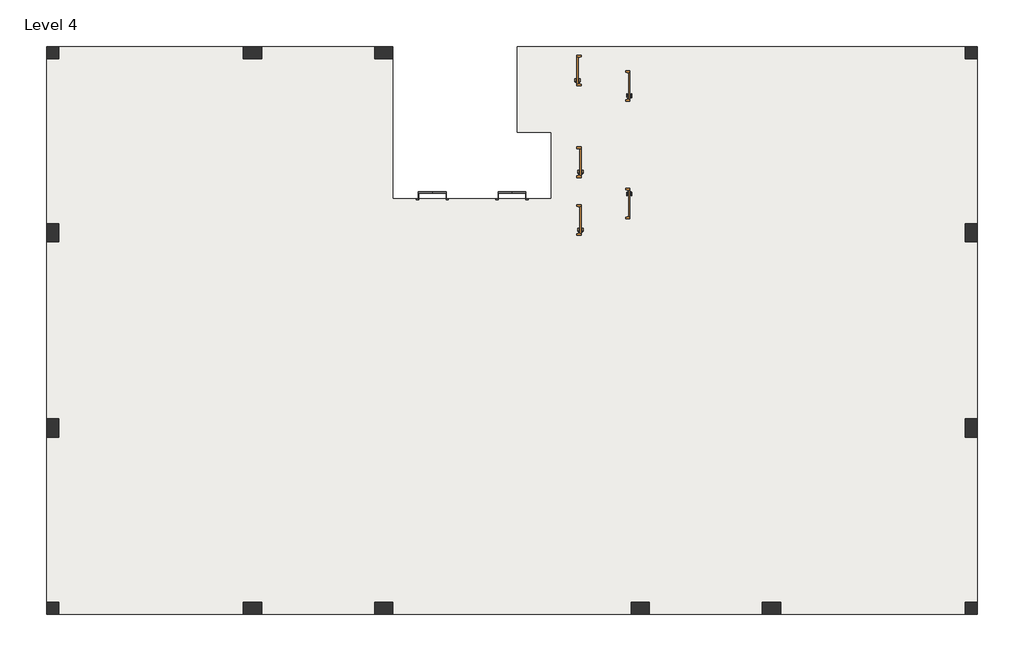
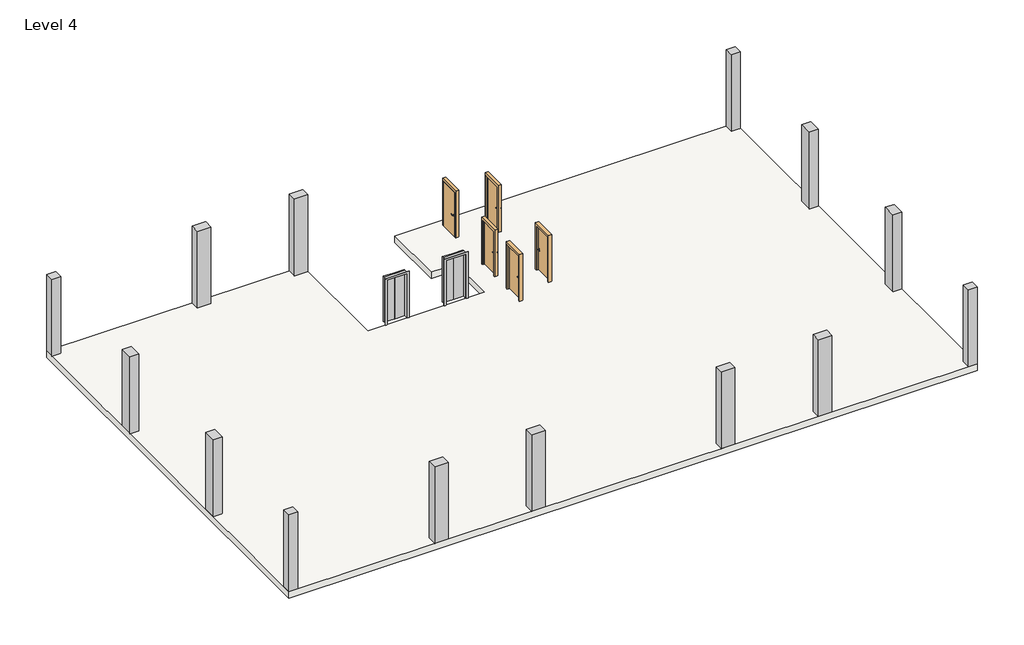
# One storey: 14 columns, 5 doors, 2 proxies, 1 slab.
"""IFC4 building model written with IfcOpenShell, lengths in millimetres."""

import ifcopenshell
import ifcopenshell.guid

model = None  # the IFC model being written
_history = None  # IfcOwnerHistory: only IFC2X3 demands one
_inside = {}  # id of a spatial element -> (the spatial element, [elements in it])
_under = {}  # id of a project, library or spatial element -> (it, [spatial elements below it])
_declared = {}  # id of a project -> (the project, [libraries it declares])
_typed = {}  # id of a type object -> (the type object, [elements of that type])
_made_of = {}  # id of a material, layer set ... -> (it, [elements and type objects made of it])


def new_model(schema):
    """Start an empty IFC model of exactly this schema.

    Asked for "IFC4X3", IfcOpenShell would pick the latest addendum, in which some entities
    have other attributes; the version numbers below select the first issue.
    IFC2X3 requires an IfcOwnerHistory on every rooted entity: one is made here for all.
    """
    global model, _history
    if schema == "IFC4X3":
        model = ifcopenshell.file(schema_version=(4, 3, 0, 0))
    else:
        model = ifcopenshell.file(schema=schema)
    _inside.clear()
    _under.clear()
    _declared.clear()
    _typed.clear()
    _made_of.clear()
    _history = None
    if model.schema == "IFC2X3":
        org = make("IfcOrganization", Name="unknown")
        user = make(
            "IfcPersonAndOrganization",
            ThePerson=make("IfcPerson", FamilyName="unknown"),
            TheOrganization=org,
        )
        app = make(
            "IfcApplication",
            ApplicationDeveloper=org,
            Version="unknown",
            ApplicationFullName="unknown",
            ApplicationIdentifier="unknown",
        )
        _history = make(
            "IfcOwnerHistory",
            OwningUser=user,
            OwningApplication=app,
            ChangeAction="ADDED",
            CreationDate=0,
        )
    return model


def make(cls, **values):
    """One entity of the class cls with the attributes given. An attribute that is None is left unset."""
    return model.create_entity(
        cls, **{name: value for name, value in values.items() if value is not None}
    )


def rooted(cls, **values):
    """An entity with a GlobalId (a new one), such as an element, a storey or a relation."""
    return make(cls, GlobalId=ifcopenshell.guid.new(), OwnerHistory=_history, **values)


def si_unit(unit_type, name, prefix=None):
    """IfcSIUnit, for example si_unit("LENGTHUNIT", "METRE", prefix="MILLI")."""
    return make("IfcSIUnit", UnitType=unit_type, Prefix=prefix, Name=name)


def assignment(units):
    """IfcUnitAssignment: the units of a project."""
    return None if units is None else make("IfcUnitAssignment", Units=units)


def point(xyz):
    """IfcCartesianPoint."""
    return None if xyz is None else make("IfcCartesianPoint", Coordinates=xyz)


def direction(xyz):
    """IfcDirection."""
    return None if xyz is None else make("IfcDirection", DirectionRatios=xyz)


def frame(location, z_axis=None, x_axis=None):
    """IfcAxis2Placement3D, a coordinate frame: its origin and axes. An axis left out is left unset."""
    return make(
        "IfcAxis2Placement3D",
        Location=point(location),
        Axis=direction(z_axis),
        RefDirection=direction(x_axis),
    )


def frame_2d(location, x_axis=None):
    """IfcAxis2Placement2D, a coordinate frame in the plane: its origin and x axis."""
    return make(
        "IfcAxis2Placement2D", Location=point(location), RefDirection=direction(x_axis)
    )


def origin():
    """The frame at (0, 0, 0) with its axes left unset."""
    return frame((0.0, 0.0, 0.0))


def origin_with_axes():
    """The frame at (0, 0, 0) with the z axis (0, 0, 1) and the x axis (1, 0, 0) written out."""
    return frame((0.0, 0.0, 0.0), z_axis=(0.0, 0.0, 1.0), x_axis=(1.0, 0.0, 0.0))


def place(relative_to, where):
    """IfcLocalPlacement: puts the frame where relative to a parent placement (None: the world)."""
    return make(
        "IfcLocalPlacement", PlacementRelTo=relative_to, RelativePlacement=where
    )


def context(
    kind, dimensions, precision=None, world=None, true_north=None, identifier=None
):
    """IfcGeometricRepresentationContext, for example the 3D "Model" context."""
    return make(
        "IfcGeometricRepresentationContext",
        ContextIdentifier=identifier,
        ContextType=kind,
        CoordinateSpaceDimension=dimensions,
        Precision=precision,
        WorldCoordinateSystem=world,
        TrueNorth=true_north,
    )


def project(units=None, contexts=None):
    """IfcProject with its units and contexts."""
    return rooted(
        "IfcProject",
        Name="project",
        RepresentationContexts=contexts,
        UnitsInContext=assignment(units),
    )


def spatial(cls, under=None, at=None, **own):
    """A site, building, storey or space (cls), placed at a placement, below another one or the project."""
    s = rooted(cls, ObjectPlacement=at, **own)
    if under is not None:
        _under.setdefault(under.id(), (under, []))[1].append(s)
    return s


def polyline(points):
    """IfcPolyline through the points."""
    return make("IfcPolyline", Points=[point(p) for p in points])


def circle_curve(where, radius):
    """IfcCircle in the frame where."""
    return make("IfcCircle", Position=where, Radius=radius)


def ellipse_curve(where, semi_axis1, semi_axis2):
    """IfcEllipse in the frame where."""
    return make(
        "IfcEllipse", Position=where, SemiAxis1=semi_axis1, SemiAxis2=semi_axis2
    )


def trimmed(basis, trim1, trim2, sense, master):
    """IfcTrimmedCurve: the piece of a basis curve between two trims."""
    return make(
        "IfcTrimmedCurve",
        BasisCurve=basis,
        Trim1=trim1,
        Trim2=trim2,
        SenseAgreement=sense,
        MasterRepresentation=master,
    )


def segment(curve, same_sense, transition):
    """IfcCompositeCurveSegment."""
    return make(
        "IfcCompositeCurveSegment",
        Transition=transition,
        SameSense=same_sense,
        ParentCurve=curve,
    )


def composite_curve(segments, self_intersect=None):
    """IfcCompositeCurve: segments joined end to end."""
    return make("IfcCompositeCurve", Segments=segments, SelfIntersect=self_intersect)


def outline(outer, holes=None, kind="AREA"):
    """IfcArbitraryClosedProfileDef: a profile drawn as a closed curve; with holes, ...WithVoids."""
    if holes is None:
        return make("IfcArbitraryClosedProfileDef", ProfileType=kind, OuterCurve=outer)
    return make(
        "IfcArbitraryProfileDefWithVoids",
        ProfileType=kind,
        OuterCurve=outer,
        InnerCurves=holes,
    )


def extrude(swept, where, along, depth):
    """IfcExtrudedAreaSolid: the profile swept, set in the frame where, extruded along a direction by depth."""
    return make(
        "IfcExtrudedAreaSolid",
        SweptArea=swept,
        Position=where,
        ExtrudedDirection=direction(along),
        Depth=depth,
    )


def faces_of(points, faces, orient=None, outer=None):
    """IfcFace entities. A face is a list of loops; a loop is a list of indices into points, from 0.

    orient and outer hold one flag for each loop. By default every Orientation is true, the
    first loop of a face is its IfcFaceOuterBound and the others are IfcFaceBound.
    """
    made = []
    for i, loops in enumerate(faces):
        bounds = []
        for j, loop in enumerate(loops):
            is_outer = j == 0 if outer is None else outer[i][j]
            bounds.append(
                make(
                    "IfcFaceOuterBound" if is_outer else "IfcFaceBound",
                    Bound=make("IfcPolyLoop", Polygon=[points[k] for k in loop]),
                    Orientation=True if orient is None else orient[i][j],
                )
            )
        made.append(make("IfcFace", Bounds=bounds))
    return made


def faceted_brep(points, faces, orient=None, outer=None, voids=None):
    """IfcFacetedBrep: a solid bounded by flat faces; with voids (closed shells), ...WithVoids."""
    shared = [point(p) for p in points]
    hull = make("IfcClosedShell", CfsFaces=faces_of(shared, faces, orient, outer))
    if voids is None:
        return make("IfcFacetedBrep", Outer=hull)
    return make(
        "IfcFacetedBrepWithVoids",
        Outer=hull,
        Voids=[
            make(cls, CfsFaces=faces_of(shared, fs, o, b)) for cls, fs, o, b in voids
        ],
    )


def shape(context_of_items, identifier, shape_type, items):
    """IfcShapeRepresentation: the items that make up one representation, for example the "Body"."""
    return make(
        "IfcShapeRepresentation",
        ContextOfItems=context_of_items,
        RepresentationIdentifier=identifier,
        RepresentationType=shape_type,
        Items=items,
    )


def source(mapping_origin, context_of_items, identifier, shape_type, items):
    """IfcRepresentationMap: a shape defined once, which mapped items show again and again."""
    return make(
        "IfcRepresentationMap",
        MappingOrigin=mapping_origin,
        MappedRepresentation=shape(context_of_items, identifier, shape_type, items),
    )


def transform(
    local_origin,
    x_axis=None,
    y_axis=None,
    z_axis=None,
    scale=None,
    scale2=None,
    scale3=None,
    uniform=True,
):
    """IfcCartesianTransformationOperator3D, or its non-uniform kind. x_axis, y_axis, z_axis: its Axis1, 2, 3."""
    if uniform:
        return make(
            "IfcCartesianTransformationOperator3D",
            Axis1=direction(x_axis),
            Axis2=direction(y_axis),
            LocalOrigin=point(local_origin),
            Scale=scale,
            Axis3=direction(z_axis),
        )
    return make(
        "IfcCartesianTransformationOperator3DnonUniform",
        Axis1=direction(x_axis),
        Axis2=direction(y_axis),
        LocalOrigin=point(local_origin),
        Scale=scale,
        Axis3=direction(z_axis),
        Scale2=scale2,
        Scale3=scale3,
    )


def mapped(mapping_source, mapping_target):
    """IfcMappedItem: shows the shape of a source again, moved by a transform."""
    return make(
        "IfcMappedItem", MappingSource=mapping_source, MappingTarget=mapping_target
    )


def made_of(thing, what):
    """Note that an element or type object is made of a material, layer set ...; save() writes the relation."""
    if what is not None:
        _made_of.setdefault(what.id(), (what, []))[1].append(thing)
    return thing


def element(
    cls,
    number,
    at=None,
    inside=None,
    cuts=None,
    type_object=None,
    material=None,
    context=None,
    identifier="Body",
    shape_type=None,
    held_by="IfcProductDefinitionShape",
    body=None,
    shapes=None,
    **own,
):
    """One element of the class cls, such as IfcWall. Its Tag is "e" and its number.

    at: its placement. inside: the storey or other place that contains it. cuts: it is an
    opening in that element (IfcRelVoidsElement). A single representation is given by context,
    identifier, shape_type and body (its items); several are given by shapes. held_by: the class
    of the entity that holds the representations. save() writes the other relations.
    """
    e = rooted(cls, Tag="e%d" % number, ObjectPlacement=at, **own)
    if body is not None:
        shapes = [shape(context, identifier, shape_type, body)]
    if shapes is not None:
        e.Representation = make(held_by, Representations=shapes)
    if inside is not None:
        _inside.setdefault(inside.id(), (inside, []))[1].append(e)
    if cuts is not None:
        rooted(
            "IfcRelVoidsElement", RelatingBuildingElement=cuts, RelatedOpeningElement=e
        )
    if type_object is not None:
        _typed.setdefault(type_object.id(), (type_object, []))[1].append(e)
    return made_of(e, material)


def aggregate(whole, parts):
    """IfcRelAggregates: a whole, such as a stair, and the parts it consists of."""
    return rooted("IfcRelAggregates", RelatingObject=whole, RelatedObjects=parts)


def save(model, path):
    """Write the relations noted so far, then the file.

    IfcRelAggregates (storeys below a building ...), IfcRelContainedInSpatialStructure (elements
    in a storey), IfcRelDefinesByType, IfcRelAssociatesMaterial and IfcRelDeclares: one each for
    every whole, place, type object, material and project.
    """
    for whole, parts in _under.values():
        aggregate(whole, parts)
    for where, things in _inside.values():
        rooted(
            "IfcRelContainedInSpatialStructure",
            RelatedElements=things,
            RelatingStructure=where,
        )
    for kind, things in _typed.values():
        rooted("IfcRelDefinesByType", RelatedObjects=things, RelatingType=kind)
    for what, things in _made_of.values():
        rooted("IfcRelAssociatesMaterial", RelatedObjects=things, RelatingMaterial=what)
    for by, libraries in _declared.values():
        rooted("IfcRelDeclares", RelatingContext=by, RelatedDefinitions=libraries)
    model.write(path)


def plane_surface(at):
    """IfcPlane: the flat surface through the origin of the frame at, square to its z axis."""
    return make("IfcPlane", Position=at)


def cylinder_surface(at, radius):
    """IfcCylindricalSurface: all points at the distance radius from the z axis of the frame at."""
    return make("IfcCylindricalSurface", Position=at, Radius=radius)


def revolved_surface(curve, axis_point, axis_direction):
    """IfcSurfaceOfRevolution: the curve turned about the line through axis_point along axis_direction."""
    return make(
        "IfcSurfaceOfRevolution",
        SweptCurve=make("IfcArbitraryOpenProfileDef", ProfileType="CURVE", Curve=curve),
        AxisPosition=make("IfcAxis1Placement", Location=point(axis_point), Axis=direction(axis_direction)),
    )


def advanced_brep(points, edges, surfaces, faces):
    """IfcAdvancedBrep: a solid bounded by faces that lie on surfaces and meet in shared edges.

    An edge is (start, end): straight between two places in points (the first is 0);
    or (start, end, curve); or (start, end, curve, False) where it runs against its curve.
    A face is (place in surfaces, loops), or (place, loops, False) where it looks against
    its surface's normal. A loop lists edges by number (the first is 1), with a minus sign
    where the edge is run from its end to its start. The first loop is the outer one.
    """
    corners = [point(p) for p in points]
    vertices = [make("IfcVertexPoint", VertexGeometry=c) for c in corners]
    made = []
    for start, end, *more in edges:
        made.append(
            make(
                "IfcEdgeCurve",
                EdgeStart=vertices[start],
                EdgeEnd=vertices[end],
                EdgeGeometry=more[0] if more else make("IfcPolyline", Points=[corners[start], corners[end]]),
                SameSense=more[1] if len(more) > 1 else True,
            )
        )
    hull = []
    for where, loops, *sense in faces:
        bounds = []
        for j, loop in enumerate(loops):
            ring = [make("IfcOrientedEdge", EdgeElement=made[abs(k) - 1], Orientation=k > 0) for k in loop]
            bounds.append(
                make(
                    "IfcFaceOuterBound" if j == 0 else "IfcFaceBound",
                    Bound=make("IfcEdgeLoop", EdgeList=ring),
                    Orientation=True,
                )
            )
        hull.append(make("IfcAdvancedFace", Bounds=bounds, FaceSurface=surfaces[where], SameSense=sense[0] if sense else True))
    return make("IfcAdvancedBrep", Outer=make("IfcClosedShell", CfsFaces=hull))


def proxy_71d7088b(model_context):
    return source(origin(), model_context, "Body", "SweptSolid", [
        extrude(outline(polyline([(-102.3106443, 96.8375), (-562.6856443, 96.8375), (-562.6856443, 147.6375), (-102.3106443, 147.6375), (-102.3106443, 96.8375)])), origin_with_axes(), (0.0, 0.0, 1.0), 2159.0),
        extrude(outline(polyline([(364.4143557, 96.8375), (-95.9606443, 96.8375), (-95.9606443, 147.6375), (364.4143557, 147.6375), (364.4143557, 96.8375)])), origin_with_axes(), (0.0, 0.0, 1.0), 2159.0),
        extrude(outline(polyline([(0.0, -562.6856443), (0.0, -556.3356443), (2133.6, -556.3356443), (2133.6, 358.0643557), (0.0, 358.0643557), (0.0, 364.4143557), (2159.0, 364.4143557), (2159.0, -562.6856443), (0.0, -562.6856443)])), frame((0.0, -96.8375, 0.0), z_axis=(0.0, 1.0, 0.0), x_axis=(0.0, 0.0, 1.0)), (0.0, 0.0, 1.0), 193.675),
        extrude(outline(polyline([(0.0, -632.5356443), (0.0, -556.3356443), (2133.6, -556.3356443), (2133.6, 358.0643557), (0.0, 358.0643557), (0.0, 434.2643557), (2209.8, 434.2643557), (2209.8, -632.5356443), (0.0, -632.5356443)])), frame((0.0, -122.2375, 0.0), z_axis=(0.0, 1.0, 0.0), x_axis=(0.0, 0.0, 1.0)), (0.0, 0.0, 1.0), 25.4),
    ])


def door_9f6fe377(model_context):
    return source(origin(), model_context, "Body", "SolidModel", [
        advanced_brep(
        [(-392.190625, -25.3375, 1016.0), (-372.190625, -25.3375, 1016.0), (-392.190625, 4.6625, 1016.0), (-372.190625, 4.6625, 1016.0), (-367.190625, 9.6625, 1016.0), (-367.190625, 29.6625, 1016.0), (-262.190625, 29.6625, 1016.0), (-262.190625, 9.6625, 1016.0)],
        [
            (0, 1, circle_curve(frame((-382.190625, -25.3375, 1016.0), z_axis=(0.0, -1.0, 0.0), x_axis=(1.0, 0.0, 0.0)), 10.0)),
            (1, 0, circle_curve(frame((-382.190625, -25.3375, 1016.0), z_axis=(0.0, -1.0, 0.0), x_axis=(1.0, 0.0, 0.0)), 10.0)),
            (0, 2),
            (2, 3, circle_curve(frame((-382.190625, 4.6625, 1016.0), z_axis=(0.0, -1.0, 0.0), x_axis=(1.0, 0.0, 0.0)), 10.0)),
            (3, 1),
            (3, 2, circle_curve(frame((-382.190625, 4.6625, 1016.0), z_axis=(0.0, -1.0, 0.0), x_axis=(1.0, 0.0, 0.0)), 10.0)),
            (4, 3, circle_curve(frame((-367.190625, 4.6625, 1016.0), z_axis=(0.0, 0.0, 1.0), x_axis=(-1.0, 0.0, 0.0)), 5.0)),
            (2, 5, circle_curve(frame((-367.190625, 4.6625, 1016.0), z_axis=(0.0, 0.0, -1.0), x_axis=(-1.0, 0.0, 0.0)), 25.0)),
            (5, 4, circle_curve(frame((-367.190625, 19.6625, 1016.0), z_axis=(-1.0, 0.0, 0.0), x_axis=(0.0, -1.0, 0.0)), 10.0)),
            (4, 5, circle_curve(frame((-367.190625, 19.6625, 1016.0), z_axis=(-1.0, 0.0, 0.0), x_axis=(0.0, -1.0, 0.0)), 10.0)),
            (6, 7, circle_curve(frame((-262.190625, 19.6625, 1016.0), z_axis=(1.0, 0.0, 0.0), x_axis=(0.0, -1.0, 0.0)), 10.0)),
            (7, 6, circle_curve(frame((-262.190625, 19.6625, 1016.0), z_axis=(1.0, 0.0, 0.0), x_axis=(0.0, -1.0, 0.0)), 10.0)),
            (5, 6),
            (7, 4),
        ],
        [
            plane_surface(frame((-382.190625, -25.3375, 1016.0), z_axis=(0.0, -1.0, 0.0), x_axis=(0.0, 0.0, 1.0))),
            cylinder_surface(frame((-382.190625, -25.3375, 1016.0), z_axis=(0.0, -1.0, 0.0), x_axis=(1.0, 0.0, 0.0)), 10.0),
            revolved_surface(trimmed(ellipse_curve(frame((-382.190625, 4.6625, 1016.0), z_axis=(0.0, -1.0, 0.0), x_axis=(1.0, 0.0, 0.0)), 10.0, 10.0), [point((-392.190625, 4.6625, 1016.0))], [point((-372.190625, 4.6625, 1016.0))], True, "CARTESIAN"), (-367.190625, 4.6625, 1016.0), (0.0, 0.0, -1.0)),
            revolved_surface(trimmed(ellipse_curve(frame((-382.190625, 4.6625, 1016.0), z_axis=(0.0, -1.0, 0.0), x_axis=(1.0, 0.0, 0.0)), 10.0, 10.0), [point((-372.190625, 4.6625, 1016.0))], [point((-392.190625, 4.6625, 1016.0))], True, "CARTESIAN"), (-367.190625, 4.6625, 1016.0), (0.0, 0.0, -1.0)),
            plane_surface(frame((-262.190625, 19.6625, 1016.0), z_axis=(1.0, 0.0, 0.0), x_axis=(0.0, 0.0, 1.0))),
            cylinder_surface(frame((-367.190625, 19.6625, 1016.0), z_axis=(-1.0, 0.0, 0.0), x_axis=(0.0, -1.0, 0.0)), 10.0),
        ],
        [
            (0, [[1, 2]]),
            (1, [[-1, 3, 4, 5]]),
            (1, [[-2, -5, 6, -3]]),
            (2, [[7, -4, 8, 9]]),
            (3, [[-8, -6, -7, 10]]),
            (4, [[11, 12]]),
            (5, [[-9, 13, -12, 14]]),
            (5, [[-10, -14, -11, -13]]),
        ],
    ),
        extrude(outline(composite_curve([segment(trimmed(circle_curve(frame_2d((1016.0, -384.690625)), 30.0), [point((1016.0, -414.690625))], [point((1016.0, -354.690625))], False, "CARTESIAN"), True, "CONTINUOUS"), segment(trimmed(circle_curve(frame_2d((1016.0, -384.690625)), 30.0), [point((1016.0, -354.690625))], [point((1016.0, -414.690625))], False, "CARTESIAN"), True, "CONTINUOUS")], self_intersect=False)), frame((0.0, -33.3375, 0.0), z_axis=(0.0, 1.0, 0.0), x_axis=(0.0, 0.0, 1.0)), (0.0, 0.0, 1.0), 8.0),
        advanced_brep(
        [(-392.190625, -85.7875, 1016.0), (-372.190625, -85.7875, 1016.0), (-372.190625, -115.7875, 1016.0), (-392.190625, -115.7875, 1016.0), (-367.190625, -120.7875, 1016.0), (-367.190625, -140.7875, 1016.0), (-262.190625, -140.7875, 1016.0), (-262.190625, -120.7875, 1016.0)],
        [
            (0, 1, circle_curve(frame((-382.190625, -85.7875, 1016.0), z_axis=(0.0, 1.0, 0.0), x_axis=(1.0, 0.0, 0.0)), 10.0)),
            (1, 0, circle_curve(frame((-382.190625, -85.7875, 1016.0), z_axis=(0.0, 1.0, 0.0), x_axis=(1.0, 0.0, 0.0)), 10.0)),
            (1, 2),
            (2, 3, circle_curve(frame((-382.190625, -115.7875, 1016.0), z_axis=(0.0, 1.0, 0.0), x_axis=(1.0, 0.0, 0.0)), 10.0)),
            (3, 0),
            (3, 2, circle_curve(frame((-382.190625, -115.7875, 1016.0), z_axis=(0.0, 1.0, 0.0), x_axis=(1.0, 0.0, 0.0)), 10.0)),
            (4, 5, circle_curve(frame((-367.190625, -130.7875, 1016.0), z_axis=(-1.0, 0.0, 0.0), x_axis=(0.0, 1.0, 0.0)), 10.0)),
            (5, 3, circle_curve(frame((-367.190625, -115.7875, 1016.0), z_axis=(0.0, 0.0, -1.0), x_axis=(-1.0, 0.0, 0.0)), 25.0)),
            (2, 4, circle_curve(frame((-367.190625, -115.7875, 1016.0), z_axis=(0.0, 0.0, 1.0), x_axis=(-1.0, 0.0, 0.0)), 5.0)),
            (5, 4, circle_curve(frame((-367.190625, -130.7875, 1016.0), z_axis=(-1.0, 0.0, 0.0), x_axis=(0.0, 1.0, 0.0)), 10.0)),
            (6, 7, circle_curve(frame((-262.190625, -130.7875, 1016.0), z_axis=(1.0, 0.0, 0.0), x_axis=(0.0, 1.0, 0.0)), 10.0)),
            (7, 6, circle_curve(frame((-262.190625, -130.7875, 1016.0), z_axis=(1.0, 0.0, 0.0), x_axis=(0.0, 1.0, 0.0)), 10.0)),
            (4, 7),
            (6, 5),
        ],
        [
            plane_surface(frame((-382.190625, -85.7875, 1016.0), z_axis=(0.0, 1.0, 0.0), x_axis=(0.0, 0.0, 1.0))),
            cylinder_surface(frame((-382.190625, -85.7875, 1016.0), z_axis=(0.0, 1.0, 0.0), x_axis=(1.0, 0.0, 0.0)), 10.0),
            revolved_surface(trimmed(ellipse_curve(frame((-382.190625, -115.7875, 1016.0), z_axis=(0.0, -1.0, 0.0), x_axis=(1.0, 0.0, 0.0)), 10.0, 10.0), [point((-392.190625, -115.7875, 1016.0))], [point((-372.190625, -115.7875, 1016.0))], True, "CARTESIAN"), (-367.190625, -115.7875, 1016.0), (0.0, 0.0, -1.0)),
            revolved_surface(trimmed(ellipse_curve(frame((-382.190625, -115.7875, 1016.0), z_axis=(0.0, -1.0, 0.0), x_axis=(1.0, 0.0, 0.0)), 10.0, 10.0), [point((-372.190625, -115.7875, 1016.0))], [point((-392.190625, -115.7875, 1016.0))], True, "CARTESIAN"), (-367.190625, -115.7875, 1016.0), (0.0, 0.0, -1.0)),
            plane_surface(frame((-262.190625, -130.7875, 1016.0), z_axis=(1.0, 0.0, 0.0), x_axis=(0.0, 0.0, 1.0))),
            cylinder_surface(frame((-367.190625, -130.7875, 1016.0), z_axis=(-1.0, 0.0, 0.0), x_axis=(0.0, 1.0, 0.0)), 10.0),
        ],
        [
            (0, [[1, 2]]),
            (1, [[3, 4, 5, -2]]),
            (1, [[-5, 6, -3, -1]]),
            (2, [[7, 8, -4, 9]]),
            (3, [[10, -9, -6, -8]]),
            (4, [[11, 12]]),
            (5, [[13, -11, 14, -7]]),
            (5, [[-14, -12, -13, -10]]),
        ],
    ),
        extrude(outline(composite_curve([segment(trimmed(circle_curve(frame_2d((1016.0, -384.690625)), 30.0), [point((1016.0, -414.690625))], [point((1016.0, -354.690625))], False, "CARTESIAN"), True, "CONTINUOUS"), segment(trimmed(circle_curve(frame_2d((1016.0, -384.690625)), 30.0), [point((1016.0, -354.690625))], [point((1016.0, -414.690625))], False, "CARTESIAN"), True, "CONTINUOUS")], self_intersect=False)), frame((0.0, -85.7875, 0.0), z_axis=(0.0, 1.0, 0.0), x_axis=(0.0, 0.0, 1.0)), (0.0, 0.0, 1.0), 8.0),
        faceted_brep([(457.2, -28.575, 0.0), (441.325, -28.575, 0.0), (441.325, 19.05, 0.0), (457.2, 19.05, 0.0), (457.2, 68.2625, 0.0), (508.0, 68.2625, 0.0), (508.0, -77.7875, 0.0), (457.2, -77.7875, 0.0), (457.2, -77.7875, 2133.6), (457.2, -28.575, 2133.6), (508.0, -77.7875, 2235.2), (-508.0, -77.7875, 2235.2), (-508.0, -77.7875, 0.0), (-457.2, -77.7875, 0.0), (-457.2, -77.7875, 2133.6), (508.0, 68.2625, 2235.2), (457.2, 68.2625, 2133.6), (-457.2, 68.2625, 2133.6), (-457.2, 68.2625, 0.0), (-508.0, 68.2625, 0.0), (-508.0, 68.2625, 2235.2), (457.2, 19.05, 2133.6), (441.325, 19.05, 2117.725), (-441.325, 19.05, 2117.725), (-441.325, 19.05, 0.0), (-457.2, 19.05, 0.0), (-457.2, 19.05, 2133.6), (441.325, -28.575, 2117.725), (-457.2, -28.575, 2133.6), (-457.2, -28.575, 0.0), (-441.325, -28.575, 0.0), (-441.325, -28.575, 2117.725)], [[[0, 1, 2, 3, 4, 5, 6, 7]], [[7, 8, 9, 0]], [[6, 10, 11, 12, 13, 14, 8, 7]], [[5, 15, 10, 6]], [[4, 16, 17, 18, 19, 20, 15, 5]], [[3, 21, 16, 4]], [[2, 22, 23, 24, 25, 26, 21, 3]], [[1, 27, 22, 2]], [[0, 9, 28, 29, 30, 31, 27, 1]], [[8, 14, 28, 9]], [[16, 21, 26, 17]], [[22, 27, 31, 23]], [[12, 19, 18, 25, 24, 30, 29, 13]], [[13, 29, 28, 14]], [[11, 20, 19, 12]], [[17, 26, 25, 18]], [[23, 31, 30, 24]], [[15, 20, 11, 10]]]),
        extrude(outline(polyline([(457.2, -33.3375), (457.2, -77.7875), (-457.2, -77.7875), (-457.2, -33.3375), (457.2, -33.3375)])), origin_with_axes(), (0.0, 0.0, 1.0), 2133.6),
    ])


def door_87fe937e(model_context):
    return source(origin(), model_context, "Body", "SolidModel", [
        advanced_brep(
        [(-392.190625, 25.3375, 1016.0), (-372.190625, 25.3375, 1016.0), (-372.190625, -4.6625, 1016.0), (-392.190625, -4.6625, 1016.0), (-367.190625, -9.6625, 1016.0), (-367.190625, -29.6625, 1016.0), (-262.190625, -29.6625, 1016.0), (-262.190625, -9.6625, 1016.0)],
        [
            (0, 1, circle_curve(frame((-382.190625, 25.3375, 1016.0), z_axis=(0.0, 1.0, 0.0), x_axis=(1.0, 0.0, 0.0)), 10.0)),
            (1, 0, circle_curve(frame((-382.190625, 25.3375, 1016.0), z_axis=(0.0, 1.0, 0.0), x_axis=(1.0, 0.0, 0.0)), 10.0)),
            (1, 2),
            (2, 3, circle_curve(frame((-382.190625, -4.6625, 1016.0), z_axis=(0.0, 1.0, 0.0), x_axis=(1.0, 0.0, 0.0)), 10.0)),
            (3, 0),
            (3, 2, circle_curve(frame((-382.190625, -4.6625, 1016.0), z_axis=(0.0, 1.0, 0.0), x_axis=(1.0, 0.0, 0.0)), 10.0)),
            (4, 5, circle_curve(frame((-367.190625, -19.6625, 1016.0), z_axis=(-1.0, 0.0, 0.0), x_axis=(0.0, 1.0, 0.0)), 10.0)),
            (5, 3, circle_curve(frame((-367.190625, -4.6625, 1016.0), z_axis=(0.0, 0.0, -1.0), x_axis=(-1.0, 0.0, 0.0)), 25.0)),
            (2, 4, circle_curve(frame((-367.190625, -4.6625, 1016.0), z_axis=(0.0, 0.0, 1.0), x_axis=(-1.0, 0.0, 0.0)), 5.0)),
            (5, 4, circle_curve(frame((-367.190625, -19.6625, 1016.0), z_axis=(-1.0, 0.0, 0.0), x_axis=(0.0, 1.0, 0.0)), 10.0)),
            (6, 7, circle_curve(frame((-262.190625, -19.6625, 1016.0), z_axis=(1.0, 0.0, 0.0), x_axis=(0.0, 1.0, 0.0)), 10.0)),
            (7, 6, circle_curve(frame((-262.190625, -19.6625, 1016.0), z_axis=(1.0, 0.0, 0.0), x_axis=(0.0, 1.0, 0.0)), 10.0)),
            (4, 7),
            (6, 5),
        ],
        [
            plane_surface(frame((-382.190625, 25.3375, 1016.0), z_axis=(0.0, 1.0, 0.0), x_axis=(0.0, 0.0, 1.0))),
            cylinder_surface(frame((-382.190625, 25.3375, 1016.0), z_axis=(0.0, 1.0, 0.0), x_axis=(1.0, 0.0, 0.0)), 10.0),
            revolved_surface(trimmed(ellipse_curve(frame((-382.190625, -4.6625, 1016.0), z_axis=(0.0, -1.0, 0.0), x_axis=(1.0, 0.0, 0.0)), 10.0, 10.0), [point((-392.190625, -4.6625, 1016.0))], [point((-372.190625, -4.6625, 1016.0))], True, "CARTESIAN"), (-367.190625, -4.6625, 1016.0), (0.0, 0.0, -1.0)),
            revolved_surface(trimmed(ellipse_curve(frame((-382.190625, -4.6625, 1016.0), z_axis=(0.0, -1.0, 0.0), x_axis=(1.0, 0.0, 0.0)), 10.0, 10.0), [point((-372.190625, -4.6625, 1016.0))], [point((-392.190625, -4.6625, 1016.0))], True, "CARTESIAN"), (-367.190625, -4.6625, 1016.0), (0.0, 0.0, -1.0)),
            plane_surface(frame((-262.190625, -19.6625, 1016.0), z_axis=(1.0, 0.0, 0.0), x_axis=(0.0, 0.0, 1.0))),
            cylinder_surface(frame((-367.190625, -19.6625, 1016.0), z_axis=(-1.0, 0.0, 0.0), x_axis=(0.0, 1.0, 0.0)), 10.0),
        ],
        [
            (0, [[1, 2]]),
            (1, [[3, 4, 5, -2]]),
            (1, [[-5, 6, -3, -1]]),
            (2, [[7, 8, -4, 9]]),
            (3, [[10, -9, -6, -8]]),
            (4, [[11, 12]]),
            (5, [[13, -11, 14, -7]]),
            (5, [[-14, -12, -13, -10]]),
        ],
    ),
        extrude(outline(composite_curve([segment(trimmed(circle_curve(frame_2d((1016.0, -384.690625)), 30.0), [point((1016.0, -414.690625))], [point((1016.0, -354.690625))], False, "CARTESIAN"), True, "CONTINUOUS"), segment(trimmed(circle_curve(frame_2d((1016.0, -384.690625)), 30.0), [point((1016.0, -354.690625))], [point((1016.0, -414.690625))], False, "CARTESIAN"), True, "CONTINUOUS")], self_intersect=False)), frame((0.0, 25.3375, 0.0), z_axis=(0.0, 1.0, 0.0), x_axis=(0.0, 0.0, 1.0)), (0.0, 0.0, 1.0), 8.0),
        advanced_brep(
        [(-392.190625, 85.7875, 1016.0), (-372.190625, 85.7875, 1016.0), (-392.190625, 115.7875, 1016.0), (-372.190625, 115.7875, 1016.0), (-367.190625, 120.7875, 1016.0), (-367.190625, 140.7875, 1016.0), (-262.190625, 140.7875, 1016.0), (-262.190625, 120.7875, 1016.0)],
        [
            (0, 1, circle_curve(frame((-382.190625, 85.7875, 1016.0), z_axis=(0.0, -1.0, 0.0), x_axis=(1.0, 0.0, 0.0)), 10.0)),
            (1, 0, circle_curve(frame((-382.190625, 85.7875, 1016.0), z_axis=(0.0, -1.0, 0.0), x_axis=(1.0, 0.0, 0.0)), 10.0)),
            (0, 2),
            (2, 3, circle_curve(frame((-382.190625, 115.7875, 1016.0), z_axis=(0.0, -1.0, 0.0), x_axis=(1.0, 0.0, 0.0)), 10.0)),
            (3, 1),
            (3, 2, circle_curve(frame((-382.190625, 115.7875, 1016.0), z_axis=(0.0, -1.0, 0.0), x_axis=(1.0, 0.0, 0.0)), 10.0)),
            (4, 3, circle_curve(frame((-367.190625, 115.7875, 1016.0), z_axis=(0.0, 0.0, 1.0), x_axis=(-1.0, 0.0, 0.0)), 5.0)),
            (2, 5, circle_curve(frame((-367.190625, 115.7875, 1016.0), z_axis=(0.0, 0.0, -1.0), x_axis=(-1.0, 0.0, 0.0)), 25.0)),
            (5, 4, circle_curve(frame((-367.190625, 130.7875, 1016.0), z_axis=(-1.0, 0.0, 0.0), x_axis=(0.0, -1.0, 0.0)), 10.0)),
            (4, 5, circle_curve(frame((-367.190625, 130.7875, 1016.0), z_axis=(-1.0, 0.0, 0.0), x_axis=(0.0, -1.0, 0.0)), 10.0)),
            (6, 7, circle_curve(frame((-262.190625, 130.7875, 1016.0), z_axis=(1.0, 0.0, 0.0), x_axis=(0.0, -1.0, 0.0)), 10.0)),
            (7, 6, circle_curve(frame((-262.190625, 130.7875, 1016.0), z_axis=(1.0, 0.0, 0.0), x_axis=(0.0, -1.0, 0.0)), 10.0)),
            (5, 6),
            (7, 4),
        ],
        [
            plane_surface(frame((-382.190625, 85.7875, 1016.0), z_axis=(0.0, -1.0, 0.0), x_axis=(0.0, 0.0, 1.0))),
            cylinder_surface(frame((-382.190625, 85.7875, 1016.0), z_axis=(0.0, -1.0, 0.0), x_axis=(1.0, 0.0, 0.0)), 10.0),
            revolved_surface(trimmed(ellipse_curve(frame((-382.190625, 115.7875, 1016.0), z_axis=(0.0, -1.0, 0.0), x_axis=(1.0, 0.0, 0.0)), 10.0, 10.0), [point((-392.190625, 115.7875, 1016.0))], [point((-372.190625, 115.7875, 1016.0))], True, "CARTESIAN"), (-367.190625, 115.7875, 1016.0), (0.0, 0.0, -1.0)),
            revolved_surface(trimmed(ellipse_curve(frame((-382.190625, 115.7875, 1016.0), z_axis=(0.0, -1.0, 0.0), x_axis=(1.0, 0.0, 0.0)), 10.0, 10.0), [point((-372.190625, 115.7875, 1016.0))], [point((-392.190625, 115.7875, 1016.0))], True, "CARTESIAN"), (-367.190625, 115.7875, 1016.0), (0.0, 0.0, -1.0)),
            plane_surface(frame((-262.190625, 130.7875, 1016.0), z_axis=(1.0, 0.0, 0.0), x_axis=(0.0, 0.0, 1.0))),
            cylinder_surface(frame((-367.190625, 130.7875, 1016.0), z_axis=(-1.0, 0.0, 0.0), x_axis=(0.0, -1.0, 0.0)), 10.0),
        ],
        [
            (0, [[1, 2]]),
            (1, [[-1, 3, 4, 5]]),
            (1, [[-2, -5, 6, -3]]),
            (2, [[7, -4, 8, 9]]),
            (3, [[-8, -6, -7, 10]]),
            (4, [[11, 12]]),
            (5, [[-9, 13, -12, 14]]),
            (5, [[-10, -14, -11, -13]]),
        ],
    ),
        extrude(outline(composite_curve([segment(trimmed(circle_curve(frame_2d((1016.0, -384.690625)), 30.0), [point((1016.0, -414.690625))], [point((1016.0, -354.690625))], False, "CARTESIAN"), True, "CONTINUOUS"), segment(trimmed(circle_curve(frame_2d((1016.0, -384.690625)), 30.0), [point((1016.0, -354.690625))], [point((1016.0, -414.690625))], False, "CARTESIAN"), True, "CONTINUOUS")], self_intersect=False)), frame((0.0, 77.7875, 0.0), z_axis=(0.0, 1.0, 0.0), x_axis=(0.0, 0.0, 1.0)), (0.0, 0.0, 1.0), 8.0),
        faceted_brep([(457.2, 28.575, 0.0), (457.2, 77.7875, 0.0), (508.0, 77.7875, 0.0), (508.0, -68.2625, 0.0), (457.2, -68.2625, 0.0), (457.2, -19.05, 0.0), (441.325, -19.05, 0.0), (441.325, 28.575, 0.0), (457.2, 28.575, 2133.6), (457.2, 77.7875, 2133.6), (-457.2, 77.7875, 2133.6), (-457.2, 77.7875, 0.0), (-508.0, 77.7875, 0.0), (-508.0, 77.7875, 2235.2), (508.0, 77.7875, 2235.2), (508.0, -68.2625, 2235.2), (-508.0, -68.2625, 2235.2), (-508.0, -68.2625, 0.0), (-457.2, -68.2625, 0.0), (-457.2, -68.2625, 2133.6), (457.2, -68.2625, 2133.6), (457.2, -19.05, 2133.6), (-457.2, -19.05, 2133.6), (-457.2, -19.05, 0.0), (-441.325, -19.05, 0.0), (-441.325, -19.05, 2117.725), (441.325, -19.05, 2117.725), (441.325, 28.575, 2117.725), (-441.325, 28.575, 2117.725), (-441.325, 28.575, 0.0), (-457.2, 28.575, 0.0), (-457.2, 28.575, 2133.6)], [[[0, 1, 2, 3, 4, 5, 6, 7]], [[1, 0, 8, 9]], [[2, 1, 9, 10, 11, 12, 13, 14]], [[3, 2, 14, 15]], [[4, 3, 15, 16, 17, 18, 19, 20]], [[5, 4, 20, 21]], [[6, 5, 21, 22, 23, 24, 25, 26]], [[7, 6, 26, 27]], [[0, 7, 27, 28, 29, 30, 31, 8]], [[9, 8, 31, 10]], [[20, 19, 22, 21]], [[26, 25, 28, 27]], [[12, 11, 30, 29, 24, 23, 18, 17]], [[11, 10, 31, 30]], [[13, 12, 17, 16]], [[19, 18, 23, 22]], [[25, 24, 29, 28]], [[15, 14, 13, 16]]]),
        extrude(outline(polyline([(457.2, 33.3375), (-457.2, 33.3375), (-457.2, 77.7875), (457.2, 77.7875), (457.2, 33.3375)])), origin_with_axes(), (0.0, 0.0, 1.0), 2133.6),
    ])


model = new_model("IFC4")

# Units and contexts
model_context = context("Model", 3, world=origin())
ifc_project = project(units=[si_unit("LENGTHUNIT", "METRE", prefix="MILLI")], contexts=[model_context])

# Site, building, storey
site = spatial("IfcSite", under=ifc_project)
building = spatial("IfcBuilding", under=site)
storey = spatial("IfcBuildingStorey", under=building, Name="Level 4", Elevation=10972.8)

# Proxies
placement = place(None, origin())
proxy_shape = proxy_71d7088b(model_context)
element("IfcBuildingElementProxy", 1, Name="Elevator Door-Center : 36\" x 84\"", ObjectType="Elevator Door-Center : 36\" x 84\"", at=placement, inside=storey, context=model_context, shape_type="MappedRepresentation", body=[
    mapped(proxy_shape, transform((-3717.8016289, 4317.8640304, 10972.8), x_axis=(1.0, 0.0, 0.0), y_axis=(0.0, 1.0, 0.0), z_axis=(0.0, 0.0, 1.0))),
])
element("IfcBuildingElementProxy", 2, Name="Elevator Door-Center : 36\" x 84\"", ObjectType="Elevator Door-Center : 36\" x 84\"", at=placement, inside=storey, context=model_context, shape_type="MappedRepresentation", body=[
    mapped(proxy_shape, transform((-1066.6766289, 4317.8640304, 10972.8), x_axis=(1.0, 0.0, 0.0), y_axis=(0.0, 1.0, 0.0), z_axis=(0.0, 0.0, 1.0))),
])

# Columns
element("IfcColumn", 3, ObjectType="Rectangular Column : 24\" x 24\"", at=placement, inside=storey, context=model_context, shape_type="SweptSolid", body=[
    extrude(outline(polyline([(-16253.4122732, 9291.5015304), (-16253.4122732, 8885.1015304), (-16659.8122732, 8885.1015304), (-16659.8122732, 9291.5015304), (-16253.4122732, 9291.5015304)])), frame((0.0, 0.0, 10972.8), z_axis=(0.0, 0.0, 1.0), x_axis=(1.0, 0.0, 0.0)), (0.0, 0.0, 1.0), 3657.6),
])
element("IfcColumn", 4, ObjectType="Rectangular Column : 24\" x 24\"", at=placement, inside=storey, context=model_context, shape_type="SweptSolid", body=[
    extrude(outline(polyline([(-16253.4122732, 3398.7015304), (-16253.4122732, 2789.1015304), (-16659.8122732, 2789.1015304), (-16659.8122732, 3398.7015304), (-16253.4122732, 3398.7015304)])), frame((0.0, 0.0, 10972.8), z_axis=(0.0, 0.0, 1.0), x_axis=(1.0, 0.0, 0.0)), (0.0, 0.0, 1.0), 3657.6),
])
element("IfcColumn", 5, ObjectType="Rectangular Column : 24\" x 24\"", at=placement, inside=storey, context=model_context, shape_type="SweptSolid", body=[
    extrude(outline(polyline([(-9497.0122732, 8885.1015304), (-10106.6122732, 8885.1015304), (-10106.6122732, 9291.5015304), (-9497.0122732, 9291.5015304), (-9497.0122732, 8885.1015304)])), frame((0.0, 0.0, 10972.8), z_axis=(0.0, 0.0, 1.0), x_axis=(1.0, 0.0, 0.0)), (0.0, 0.0, 1.0), 3657.6),
])
element("IfcColumn", 6, ObjectType="Rectangular Column : 24\" x 24\"", at=placement, inside=storey, context=model_context, shape_type="SweptSolid", body=[
    extrude(outline(polyline([(-5128.2122732, 8885.1015304), (-5737.8122732, 8885.1015304), (-5737.8122732, 9291.5015304), (-5128.2122732, 9291.5015304), (-5128.2122732, 8885.1015304)])), frame((0.0, 0.0, 10972.8), z_axis=(0.0, 0.0, 1.0), x_axis=(1.0, 0.0, 0.0)), (0.0, 0.0, 1.0), 3657.6),
])
element("IfcColumn", 7, ObjectType="Rectangular Column : 24\" x 24\"", at=placement, inside=storey, context=model_context, shape_type="SweptSolid", body=[
    extrude(outline(polyline([(14328.1877268, 8885.1015304), (13921.7877268, 8885.1015304), (13921.7877268, 9291.5015304), (14328.1877268, 9291.5015304), (14328.1877268, 8885.1015304)])), frame((0.0, 0.0, 10972.8), z_axis=(0.0, 0.0, 1.0), x_axis=(1.0, 0.0, 0.0)), (0.0, 0.0, 1.0), 3657.6),
])
element("IfcColumn", 8, ObjectType="Rectangular Column : 24\" x 24\"", at=placement, inside=storey, context=model_context, shape_type="SweptSolid", body=[
    extrude(outline(polyline([(13921.7877268, 2789.1015304), (13921.7877268, 3398.7015304), (14328.1877268, 3398.7015304), (14328.1877268, 2789.1015304), (13921.7877268, 2789.1015304)])), frame((0.0, 0.0, 10972.8), z_axis=(0.0, 0.0, 1.0), x_axis=(1.0, 0.0, 0.0)), (0.0, 0.0, 1.0), 3657.6),
])
element("IfcColumn", 9, ObjectType="Rectangular Column : 24\" x 24\"", at=placement, inside=storey, context=model_context, shape_type="SweptSolid", body=[
    extrude(outline(polyline([(13921.7877268, -3713.2984696), (13921.7877268, -3103.6984696), (14328.1877268, -3103.6984696), (14328.1877268, -3713.2984696), (13921.7877268, -3713.2984696)])), frame((0.0, 0.0, 10972.8), z_axis=(0.0, 0.0, 1.0), x_axis=(1.0, 0.0, 0.0)), (0.0, 0.0, 1.0), 3657.6),
])
element("IfcColumn", 10, ObjectType="Rectangular Column : 24\" x 24\"", at=placement, inside=storey, context=model_context, shape_type="SweptSolid", body=[
    extrude(outline(polyline([(13921.7877268, -9606.0984696), (13921.7877268, -9199.6984696), (14328.1877268, -9199.6984696), (14328.1877268, -9606.0984696), (13921.7877268, -9606.0984696)])), frame((0.0, 0.0, 10972.8), z_axis=(0.0, 0.0, 1.0), x_axis=(1.0, 0.0, 0.0)), (0.0, 0.0, 1.0), 3657.6),
])
element("IfcColumn", 11, ObjectType="Rectangular Column : 24\" x 24\"", at=placement, inside=storey, context=model_context, shape_type="SweptSolid", body=[
    extrude(outline(polyline([(7165.3877268, -9199.6984696), (7774.9877268, -9199.6984696), (7774.9877268, -9606.0984696), (7165.3877268, -9606.0984696), (7165.3877268, -9199.6984696)])), frame((0.0, 0.0, 10972.8), z_axis=(0.0, 0.0, 1.0), x_axis=(1.0, 0.0, 0.0)), (0.0, 0.0, 1.0), 3657.6),
])
element("IfcColumn", 12, ObjectType="Rectangular Column : 24\" x 24\"", at=placement, inside=storey, context=model_context, shape_type="SweptSolid", body=[
    extrude(outline(polyline([(2796.5877268, -9199.6984696), (3406.1877268, -9199.6984696), (3406.1877268, -9606.0984696), (2796.5877268, -9606.0984696), (2796.5877268, -9199.6984696)])), frame((0.0, 0.0, 10972.8), z_axis=(0.0, 0.0, 1.0), x_axis=(1.0, 0.0, 0.0)), (0.0, 0.0, 1.0), 3657.6),
])
element("IfcColumn", 13, ObjectType="Rectangular Column : 24\" x 24\"", at=placement, inside=storey, context=model_context, shape_type="SweptSolid", body=[
    extrude(outline(polyline([(-5737.8122732, -9199.6984696), (-5128.2122732, -9199.6984696), (-5128.2122732, -9606.0984696), (-5737.8122732, -9606.0984696), (-5737.8122732, -9199.6984696)])), frame((0.0, 0.0, 10972.8), z_axis=(0.0, 0.0, 1.0), x_axis=(1.0, 0.0, 0.0)), (0.0, 0.0, 1.0), 3657.6),
])
element("IfcColumn", 14, ObjectType="Rectangular Column : 24\" x 24\"", at=placement, inside=storey, context=model_context, shape_type="SweptSolid", body=[
    extrude(outline(polyline([(-10106.6122732, -9199.6984696), (-9497.0122732, -9199.6984696), (-9497.0122732, -9606.0984696), (-10106.6122732, -9606.0984696), (-10106.6122732, -9199.6984696)])), frame((0.0, 0.0, 10972.8), z_axis=(0.0, 0.0, 1.0), x_axis=(1.0, 0.0, 0.0)), (0.0, 0.0, 1.0), 3657.6),
])
element("IfcColumn", 15, ObjectType="Rectangular Column : 24\" x 24\"", at=placement, inside=storey, context=model_context, shape_type="SweptSolid", body=[
    extrude(outline(polyline([(-16659.8122732, -9199.6984696), (-16253.4122732, -9199.6984696), (-16253.4122732, -9606.0984696), (-16659.8122732, -9606.0984696), (-16659.8122732, -9199.6984696)])), frame((0.0, 0.0, 10972.8), z_axis=(0.0, 0.0, 1.0), x_axis=(1.0, 0.0, 0.0)), (0.0, 0.0, 1.0), 3657.6),
])
element("IfcColumn", 16, ObjectType="Rectangular Column : 24\" x 24\"", at=placement, inside=storey, context=model_context, shape_type="SweptSolid", body=[
    extrude(outline(polyline([(-16253.4122732, -3103.6984696), (-16253.4122732, -3713.2984696), (-16659.8122732, -3713.2984696), (-16659.8122732, -3103.6984696), (-16253.4122732, -3103.6984696)])), frame((0.0, 0.0, 10972.8), z_axis=(0.0, 0.0, 1.0), x_axis=(1.0, 0.0, 0.0)), (0.0, 0.0, 1.0), 3657.6),
])

# Doors
door_shape = door_9f6fe377(model_context)
element("IfcDoor", 17, ObjectType="Door-Passage-Single-Flush : 36\" x 84\"", at=placement, inside=storey, context=model_context, shape_type="MappedRepresentation", body=[
    mapped(door_shape, transform((1058.2752268, 5440.2265304, 10972.8), x_axis=(0.0, 1.0, 0.0), y_axis=(-1.0, 0.0, 0.0), z_axis=(0.0, 0.0, 1.0))),
])
element("IfcDoor", 18, ObjectType="Door-Passage-Single-Flush : 36\" x 84\"", at=placement, inside=storey, context=model_context, shape_type="MappedRepresentation", body=[
    mapped(door_shape, transform((1058.2752268, 3509.8265304, 10972.8), x_axis=(0.0, 1.0, 0.0), y_axis=(-1.0, 0.0, 0.0), z_axis=(0.0, 0.0, 1.0))),
])
element("IfcDoor", 19, ObjectType="Door-Passage-Single-Flush : 36\" x 84\"", at=placement, inside=storey, context=model_context, shape_type="MappedRepresentation", body=[
    mapped(door_shape, transform((2683.8752268, 7980.2265304, 10972.8), x_axis=(0.0, 1.0, 0.0), y_axis=(-1.0, 0.0, 0.0), z_axis=(0.0, 0.0, 1.0))),
])
door_2_shape = door_87fe937e(model_context)
element("IfcDoor", 20, ObjectType="Door-Passage-Single-Flush : 36\" x 84\"", at=placement, inside=storey, context=model_context, shape_type="MappedRepresentation", body=[
    mapped(door_2_shape, transform((1070.9752268, 8488.2265304, 10972.8), x_axis=(0.0, 1.0, 0.0), y_axis=(-1.0, 0.0, 0.0), z_axis=(0.0, 0.0, 1.0))),
])
element("IfcDoor", 21, ObjectType="Door-Passage-Single-Flush : 36\" x 84\"", at=placement, inside=storey, context=model_context, shape_type="MappedRepresentation", body=[
    mapped(door_2_shape, transform((2683.8752268, 4059.1015304, 10972.8), x_axis=(0.0, -1.0, 0.0), y_axis=(1.0, 0.0, 0.0), z_axis=(0.0, 0.0, 1.0))),
])

# Slab
element("IfcSlab", 22, ObjectType="Generic - 12\"", at=placement, inside=storey, context=model_context, shape_type="Brep", body=[
    faceted_brep([(14328.1877268, 9291.5015304, 10668.0), (14328.1877268, -9606.0984696, 10668.0), (-16659.8122732, -9606.0984696, 10668.0), (-16659.8122732, 9291.5015304, 10668.0), (-5128.2122732, 9291.5015304, 10668.0), (-5128.2122732, 4221.0265304, 10668.0), (-4934.5372732, 4221.0265304, 10668.0), (145.4627268, 4221.0265304, 10668.0), (145.4627268, 6446.7015304, 10668.0), (-988.0122732, 6446.7015304, 10668.0), (-988.0122732, 9291.5015304, 10668.0), (967.7877268, 9291.5015304, 10668.0), (1161.4627268, 9291.5015304, 10668.0), (2593.3877268, 9291.5015304, 10668.0), (2787.0627268, 9291.5015304, 10668.0), (8282.9877268, 9291.5015304, 10668.0), (8476.6627268, 9291.5015304, 10668.0), (14328.1877268, -9606.0984696, 10972.8), (14328.1877268, 9291.5015304, 10972.8), (8476.6627268, 9291.5015304, 10972.8), (8282.9877268, 9291.5015304, 10972.8), (2787.0627268, 9291.5015304, 10972.8), (2593.3877268, 9291.5015304, 10972.8), (1161.4627268, 9291.5015304, 10972.8), (967.7877268, 9291.5015304, 10972.8), (-988.0122732, 9291.5015304, 10972.8), (-988.0122732, 6446.7015304, 10972.8), (145.4627268, 6446.7015304, 10972.8), (145.4627268, 4221.0265304, 10972.8), (-4934.5372732, 4221.0265304, 10972.8), (-5128.2122732, 4221.0265304, 10972.8), (-5128.2122732, 9291.5015304, 10972.8), (-16659.8122732, 9291.5015304, 10972.8), (-16659.8122732, -9606.0984696, 10972.8)], [[[0, 1, 2, 3, 4, 5, 6, 7, 8, 9, 10, 11, 12, 13, 14, 15, 16]], [[17, 18, 19, 20, 21, 22, 23, 24, 25, 26, 27, 28, 29, 30, 31, 32, 33]], [[1, 0, 18, 17]], [[2, 1, 17, 33]], [[3, 2, 33, 32]], [[7, 28, 27, 8]], [[30, 5, 4, 31]], [[28, 7, 6, 5, 30, 29]], [[3, 32, 31, 4]], [[18, 0, 16, 15, 14, 13, 12, 11, 10, 25, 24, 23, 22, 21, 20, 19]], [[8, 27, 26, 9]], [[9, 26, 25, 10]]]),
])

save(model, "model.ifc")

# Revit data of these elements
# Type "Elevator Door-Center : 36\" x 84\""
#   Assembly Code = "D1010"
#   Door Height = 7' - 0"
#   Door Width = 3' - 0"
#   Trim Projection = 0' - 1"
#   Trim Width = 0' - 3"
#   Door Finish = Elevator Door
#   Frame Finish = Door - Frame
#   Default Elevation = 0
# Type "Rectangular Column : 24\" x 24\""
#   Assembly Code = "B1010200"
#   Depth = 2' - 0"
#   Offset Base = 0' - 0"
#   Offset Top = 0' - 0"
#   Width = 2' - 0"
#   Material = none
# Type "Door-Passage-Single-Flush : 36\" x 84\""
#   Type Mark = "1"
#   Assembly Code = "B2030200"
#   Analytic Construction = "Wooden"
#   Thickness = 0' - 1 3/4"
#   Thermal Resistance (R) = 2.5876 (h·ft²·°F)/BTU
#   Swing Angle [instance default] = 90.00°
#   Strike Height = 3' - 4"
#   Rough Width [instance default] = 3' - 4"
#   Rough Height [instance default] = 7' - 4"
#   MF Opening Height [instance default] = 0' - 4"
#   MF Opening Width [instance default] = 0' - 4"
#   Inset Calculate [instance default] = 0' - 4"
#   Masonry Inset [instance default] = 0' - 1"
#   Height = 7' - 0"
#   Width = 3' - 0"
#   Heat Transfer Coefficient (U) = 0.3865 BTU/(h·ft²·°F)
#   Masonry Frame Depth = 0' - 5 3/4"
#   Define Thermal Properties by = 1
#   Masonry Frame [instance default] = yes
#   Function = 1
#   Dry Wall Frame [instance default] = no
#   Panel Material = Wood - Birch
#   Frame Material = Metal - Paint Finish - Grey
#   Door Handle Material = Aluminum
#   Visual Light Transmittance = 0
#   Solar Heat Gain Coefficient = 0
#   Wall Closure = (empty or 0)
# Type "Generic - 12\""
#   Assembly Code = "B1010"
#   Function = 0
#   Layers, outside or top first: 1' - 0" no material (function 1)
# Elements 1, 2 (IfcBuildingElementProxy, "Elevator Door-Center : 36\" x 84\"")
#   Phase Created = New Construction
#   Materials on its faces: "Door - Frame", "Elevator Door"
# Elements 3, 4, 5, 6, 7, 8, 9, 10, 11, 12, 13, 14, 15, 16 (IfcColumn, "Rectangular Column : 24\" x 24\"")
#   Phase Created = New Construction
#   Materials on its faces: "Default Wall"
# Elements 17, 18, 19, 20, 21 (IfcDoor, "Door-Passage-Single-Flush : 36\" x 84\"")
#   Swing Angle = 90.00°
#   Rough Width = 3' - 4"
#   Rough Height = 7' - 4"
#   Masonry Inset = 0' - 1"
#   MF Opening Width = 0' - 4"
#   MF Opening Height = 0' - 4"
#   Inset Calculate = 0' - 4"
#   Masonry Frame = yes
#   Dry Wall Frame = no
#   Phase Created = New Construction
#   Materials on its faces: "Aluminum", "Metal - Paint Finish - Grey", "Wood - Birch"
# Element 22 (IfcSlab, "Generic - 12\"")
#   built-in parameter 1001955 = 1.5708 (stored number, unit not read)
#   Height Offset From Level = 0' - 0"
#   Phase Created = New Construction
#   Materials on its faces: "Default Floor"
# Materials
#   "Elevator Door": class "Metal", colour RGB 57 57 57, transparency 0
#   "Door - Frame": class "Miscellaneous", colour RGB 118 70 51, transparency 0, Cost = 0
#   "Wood - Birch": class "Wood", colour RGB 166 116 52, transparency 0, Cost = 0
#   "Metal - Paint Finish - Grey": class "Paint", colour RGB 104 104 104, transparency 0, Cost = 0
#   "Aluminum": class "Metal", colour RGB 247 247 247, transparency 0, Description = "Aluminum 6061", Cost = 0
#   "Default Wall": class "Miscellaneous", colour RGB 128 128 128, transparency 0, Cost = 0
#   "Default Floor": class "Miscellaneous", colour RGB 128 128 128, transparency 0, Cost = 0
